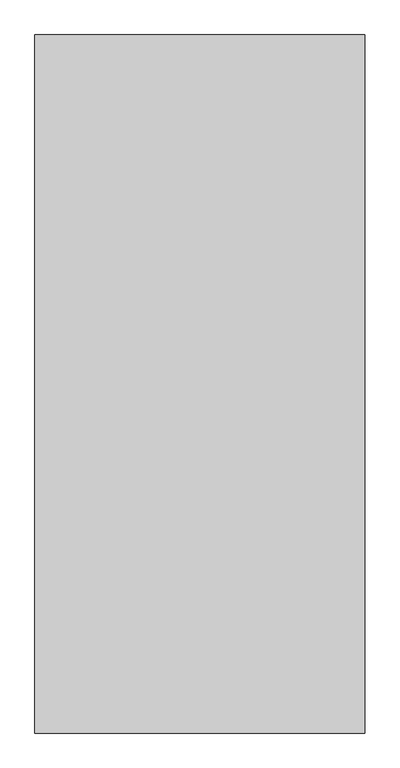
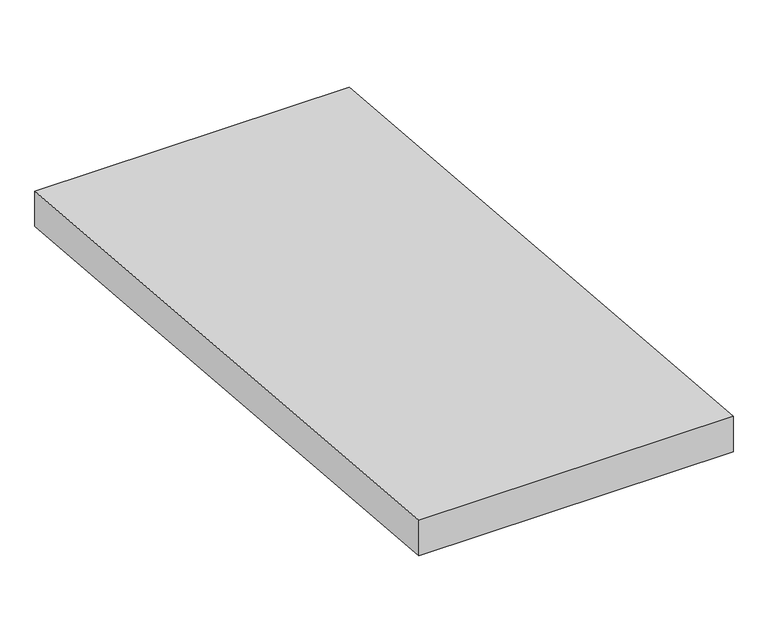
"""IFC4 building model written with IfcOpenShell, lengths in millimetres: ramp geometry."""

from ifc_helpers import new_model, si_unit, frame, origin, place, context, project, spatial, polyline, outline, extrude, source, transform, mapped, element, save


def ramp_d010aea3(model_context):
    return source(origin(), model_context, "Body", "SweptSolid", [
        extrude(outline(polyline([(19399.5208589, 149.9618634), (22999.5208589, -150.0381366), (22999.5208589, -350.7313796), (19399.5208589, -50.7313796), (19399.5208589, 149.9618634)])), frame((20675.0, 0.0, 0.0), z_axis=(1.0, 0.0, 0.0), x_axis=(0.0, 1.0, 0.0)), (0.0, 0.0, 1.0), 1700.0),
    ])


if __name__ == "__main__":
    model = new_model("IFC4")
    model_context = context("Model", 3, world=origin())
    ifc_project = project(units=[si_unit("LENGTHUNIT", "METRE", prefix="MILLI")], contexts=[model_context])
    site = spatial("IfcSite", under=ifc_project)
    building = spatial("IfcBuilding", under=site)
    placement = place(None, origin())
    ramp_shape = ramp_d010aea3(model_context)
    element("IfcRamp", 1, at=placement, inside=building, context=model_context, shape_type="MappedRepresentation", body=[
        mapped(ramp_shape, transform((0.0, 0.0, 0.0), x_axis=(1.0, 0.0, 0.0), y_axis=(0.0, 1.0, 0.0), z_axis=(0.0, 0.0, 1.0))),
    ])
    save(model, "model.ifc")

# Revit data of these elements
# Element 1 (IfcRamp)
#   Materials on its faces: "00_Concrete_Reinf. Conc."
# Materials
#   "00_Concrete_Reinf. Conc.": class "Concrete", colour RGB 176 176 176, transparency 0, Description = "Reinf. Conc.", Cost = 0, Image = Concrete.Cast-In-Place.Flat.Polished.Grey.jpg
